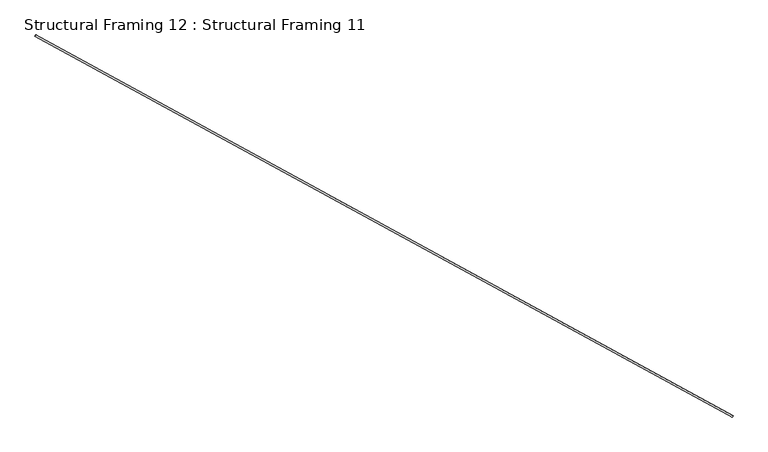
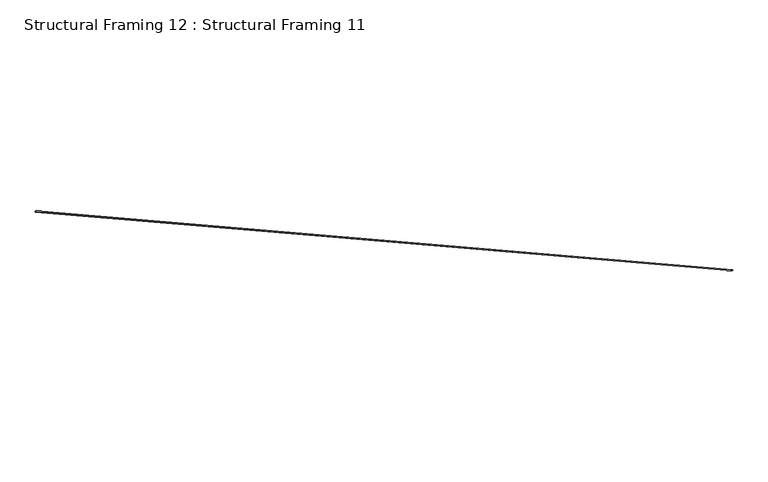
"""IFC4 building model written with IfcOpenShell, lengths in millimetres: beam geometry, Structural Framing 12 : Structural Framing 11."""

from ifc_helpers import new_model, si_unit, point, frame, origin, origin_2d, place, context, project, spatial, circle_curve, trimmed, segment, composite_curve, outline, extrude, source, transform, mapped, element, save


def structural_framing_12_structural_framing_11_33364254(model_context):
    return source(origin(), model_context, "Body", "SweptSolid", [
        extrude(outline(composite_curve([segment(trimmed(circle_curve(origin_2d(), 6.35), [point((0.0, -6.3499999))], [point((0.0, 6.35))], False, "CARTESIAN"), True, "CONTINUOUS"), segment(trimmed(circle_curve(origin_2d(), 6.35), [point((0.0, 6.35))], [point((0.0, -6.3499999))], False, "CARTESIAN"), True, "CONTINUOUS")], self_intersect=False)), frame((17939.5405771, 4177.5989868, 4934.3713104), z_axis=(-0.8714985593718706, 0.4757560037149592, 0.1189390009287357), x_axis=(0.0, -0.24253562503632659, 0.9701425001453335)), (0.0, 0.0, 1.0), 6120.4961437),
    ])


if __name__ == "__main__":
    model = new_model("IFC4")
    model_context = context("Model", 3, world=origin())
    ifc_project = project(units=[si_unit("LENGTHUNIT", "METRE", prefix="MILLI")], contexts=[model_context])
    site = spatial("IfcSite", under=ifc_project)
    building = spatial("IfcBuilding", under=site)
    placement = place(None, origin())
    structural_framing_12_structural_framing_11_shape = structural_framing_12_structural_framing_11_33364254(model_context)
    element("IfcBeam", 1, ObjectType="Structural Framing 12 : Structural Framing 11", at=placement, inside=building, context=model_context, shape_type="MappedRepresentation", body=[
        mapped(structural_framing_12_structural_framing_11_shape, transform((0.0, 0.0, 0.0), x_axis=(1.0, 0.0, 0.0), y_axis=(0.0, 1.0, 0.0), z_axis=(0.0, 0.0, 1.0))),
    ])
    save(model, "model.ifc")

# Revit data of these elements
# Type "Structural Framing 12 : Structural Framing 11"
#   Structural Material [instance default] = EXISTING LATERAL BRACING (1/4" CABLE)
# Element 1 (IfcBeam, "Structural Framing 12 : Structural Framing 11")
#   Materials on its faces: "EXISTING LATERAL BRACING (1/4\" CABLE)"
# Materials
#   "EXISTING LATERAL BRACING (1/4\" CABLE)": class "Generic", colour RGB 120 120 120, transparency 0, Cost = 0
